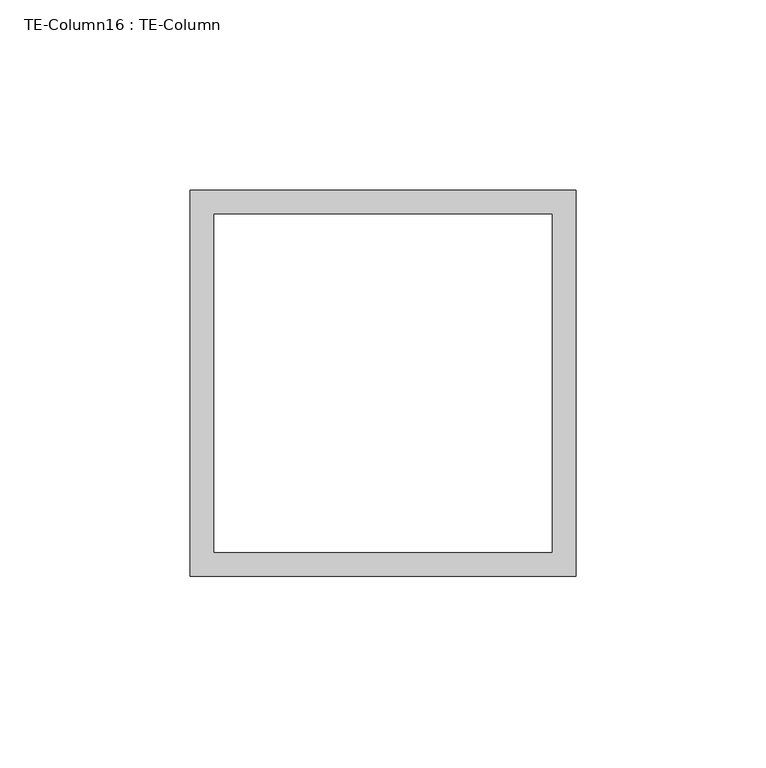
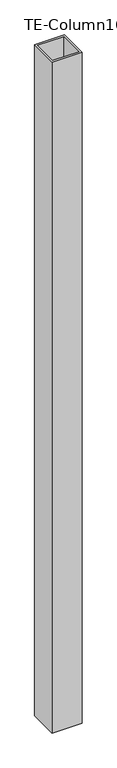
"""IFC4 building model written with IfcOpenShell, lengths in millimetres: proxy geometry, TE-Column16 : TE-Column."""

from ifc_helpers import new_model, si_unit, frame, origin, place, context, project, spatial, polyline, outline, extrude, source, transform, mapped, element, save


def te_column16_te_column_06b2476f(model_context):
    return source(origin(), model_context, "Body", "SweptSolid", [
        extrude(outline(polyline([(590318.6434739, -535255.5413841), (590217.0434739, -535255.5413841), (590217.0434739, -535153.9413841), (590318.6434739, -535153.9413841), (590318.6434739, -535255.5413841)]), holes=[polyline([(590312.2934739, -535160.2913841), (590223.3934739, -535160.2913841), (590223.3934739, -535249.1913841), (590312.2934739, -535249.1913841), (590312.2934739, -535160.2913841)])]), frame((0.0, 0.0, 28.575), z_axis=(0.0, 0.0, 1.0), x_axis=(1.0, 0.0, 0.0)), (0.0, 0.0, 1.0), 2406.65),
    ])


if __name__ == "__main__":
    model = new_model("IFC4")
    model_context = context("Model", 3, world=origin())
    ifc_project = project(units=[si_unit("LENGTHUNIT", "METRE", prefix="MILLI")], contexts=[model_context])
    site = spatial("IfcSite", under=ifc_project)
    building = spatial("IfcBuilding", under=site)
    placement = place(None, origin())
    te_column16_te_column_shape = te_column16_te_column_06b2476f(model_context)
    element("IfcBuildingElementProxy", 1, Name="TE-Column16 : TE-Column", ObjectType="TE-Column16 : TE-Column", at=placement, inside=building, context=model_context, shape_type="MappedRepresentation", body=[
        mapped(te_column16_te_column_shape, transform((0.0, 0.0, 0.0), x_axis=(1.0, 0.0, 0.0), y_axis=(0.0, 1.0, 0.0), z_axis=(0.0, 0.0, 1.0))),
    ])
    save(model, "model.ifc")

# Revit data of these elements
# Element 1 (IfcBuildingElementProxy, "TE-Column16 : TE-Column")
#   Materials on its faces: "4\"X4\" GALV. HSS TUBING"
# Materials
#   "4\"X4\" GALV. HSS TUBING": class "Generic", colour RGB 211 211 207, transparency 0, Cost = 0
